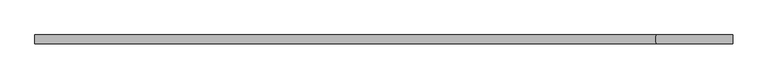
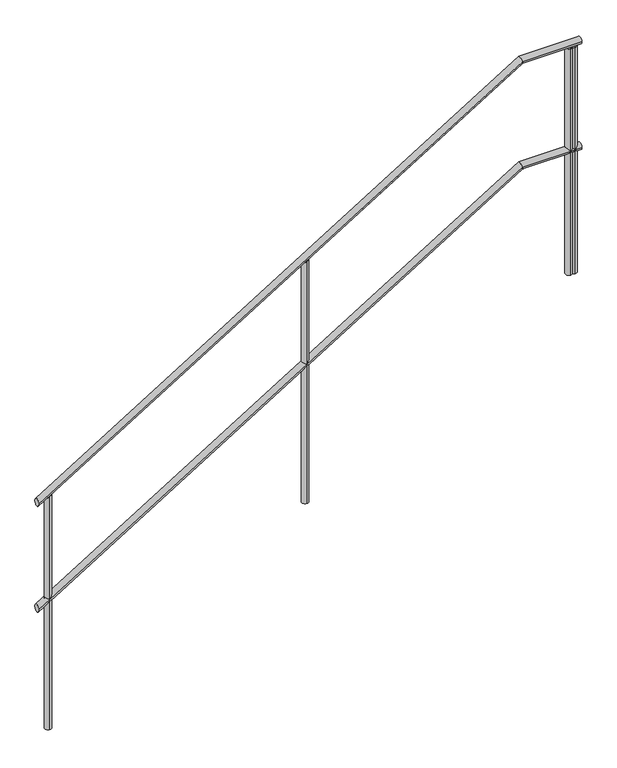
"""IFC4 building model written with IfcOpenShell, lengths in millimetres: railing geometry."""

from ifc_helpers import new_model, si_unit, point, frame, frame_2d, origin, place, context, project, spatial, circle_curve, ellipse_curve, trimmed, segment, composite_curve, outline, extrude, source, transform, mapped, element, save
from ifc_brep_helpers import plane_surface, cylinder_surface, advanced_brep


def railing_2ca88775(model_context):
    return source(origin(), model_context, "Body", "SolidModel", [
        advanced_brep(
        [(71751.0, -5865.7674116, -450.9609787), (71751.0, -5835.7674116, -450.9609787), (73915.2567855, -5835.7674116, 885.0), (73915.2567855, -5865.7674116, 885.0), (74181.0, -5865.7674116, 885.0), (74181.0, -5835.7674116, 885.0)],
        [
            (0, 1, ellipse_curve(frame((71751.0, -5850.7674116, -450.9609787), z_axis=(-1.0, 0.0, 0.0), x_axis=(0.0, 0.0, -1.0)), 17.6276454, 15.0)),
            (1, 0, ellipse_curve(frame((71751.0, -5850.7674116, -450.9609787), z_axis=(-1.0, 0.0, 0.0), x_axis=(0.0, 0.0, -1.0)), 17.6276454, 15.0)),
            (1, 2),
            (2, 3, ellipse_curve(frame((73915.2567855, -5850.7674116, 885.0), z_axis=(-0.9620125025549409, 0.0, -0.27300539358770864), x_axis=(0.27300539358770803, 0.0, -0.9620125025549412)), 15.5923129, 15.0)),
            (3, 0),
            (3, 2, ellipse_curve(frame((73915.2567855, -5850.7674116, 885.0), z_axis=(-0.9620125025549409, 0.0, -0.27300539358770864), x_axis=(0.27300539358770803, 0.0, -0.9620125025549412)), 15.5923129, 15.0)),
            (4, 5, circle_curve(frame((74181.0, -5850.7674116, 885.0), z_axis=(1.0, 0.0, 0.0), x_axis=(0.0, 1.0, 0.0)), 15.0)),
            (5, 4, circle_curve(frame((74181.0, -5850.7674116, 885.0), z_axis=(1.0, 0.0, 0.0), x_axis=(0.0, 1.0, 0.0)), 15.0)),
            (2, 5),
            (4, 3),
        ],
        [
            plane_surface(frame((71751.0, -5850.7674116, -433.3333333), z_axis=(-1.0, 0.0, 0.0), x_axis=(0.0, 1.0, 0.0))),
            cylinder_surface(frame((71758.8790381, -5850.7674116, -446.097375), z_axis=(-0.8509361101440404, 0.0, -0.5252692037926168), x_axis=(0.0, 1.0, 0.0)), 15.0),
            plane_surface(frame((74181.0, -5850.7674116, 900.0), z_axis=(1.0, 0.0, 0.0), x_axis=(0.0, 1.0, 0.0))),
            cylinder_surface(frame((73911.0, -5850.7674116, 885.0), z_axis=(-1.0, 0.0, 0.0), x_axis=(0.0, 1.0, 0.0)), 15.0),
        ],
        [
            (0, [[1, 2]]),
            (1, [[-2, 3, 4, 5]]),
            (1, [[-1, -5, 6, -3]]),
            (2, [[7, 8]]),
            (3, [[-4, 9, -7, 10]]),
            (3, [[-6, -10, -8, -9]]),
        ],
    ),
        advanced_brep(
        [(71751.0, -5865.7674116, 49.0390213), (71751.0, -5835.7674116, 49.0390213), (73915.2567855, -5835.7674116, 1385.0), (73915.2567855, -5865.7674116, 1385.0), (74181.0, -5865.7674116, 1385.0), (74181.0, -5835.7674116, 1385.0)],
        [
            (0, 1, ellipse_curve(frame((71751.0, -5850.7674116, 49.0390213), z_axis=(-1.0, 0.0, 0.0), x_axis=(0.0, 0.0, -1.0)), 17.6276454, 15.0)),
            (1, 0, ellipse_curve(frame((71751.0, -5850.7674116, 49.0390213), z_axis=(-1.0, 0.0, 0.0), x_axis=(0.0, 0.0, -1.0)), 17.6276454, 15.0)),
            (1, 2),
            (2, 3, ellipse_curve(frame((73915.2567855, -5850.7674116, 1385.0), z_axis=(-0.9620125025549409, 0.0, -0.27300539358770864), x_axis=(0.27300539358770803, 0.0, -0.9620125025549412)), 15.5923129, 15.0)),
            (3, 0),
            (3, 2, ellipse_curve(frame((73915.2567855, -5850.7674116, 1385.0), z_axis=(-0.9620125025549409, 0.0, -0.27300539358770864), x_axis=(0.27300539358770803, 0.0, -0.9620125025549412)), 15.5923129, 15.0)),
            (4, 5, circle_curve(frame((74181.0, -5850.7674116, 1385.0), z_axis=(1.0, 0.0, 0.0), x_axis=(0.0, 1.0, 0.0)), 15.0)),
            (5, 4, circle_curve(frame((74181.0, -5850.7674116, 1385.0), z_axis=(1.0, 0.0, 0.0), x_axis=(0.0, 1.0, 0.0)), 15.0)),
            (2, 5),
            (4, 3),
        ],
        [
            plane_surface(frame((71751.0, -5850.7674116, 66.6666667), z_axis=(-1.0, 0.0, 0.0), x_axis=(0.0, 1.0, 0.0))),
            cylinder_surface(frame((71758.8790381, -5850.7674116, 53.902625), z_axis=(-0.8509361101440404, 0.0, -0.5252692037926168), x_axis=(0.0, 1.0, 0.0)), 15.0),
            plane_surface(frame((74181.0, -5850.7674116, 1400.0), z_axis=(1.0, 0.0, 0.0), x_axis=(0.0, 1.0, 0.0))),
            cylinder_surface(frame((73911.0, -5850.7674116, 1385.0), z_axis=(-1.0, 0.0, 0.0), x_axis=(0.0, 1.0, 0.0)), 15.0),
        ],
        [
            (0, [[1, 2]]),
            (1, [[-2, 3, 4, 5]]),
            (1, [[-1, -5, 6, -3]]),
            (2, [[7, 8]]),
            (3, [[-4, 9, -7, 10]]),
            (3, [[-6, -10, -8, -9]]),
        ],
    ),
        extrude(outline(composite_curve([segment(trimmed(circle_curve(frame_2d((74151.0, -5850.7674116)), 15.0), [point((74151.0, -5865.7674116))], [point((74151.0, -5835.7674116))], False, "CARTESIAN"), True, "CONTINUOUS"), segment(trimmed(circle_curve(frame_2d((74151.0, -5850.7674116)), 15.0), [point((74151.0, -5835.7674116))], [point((74151.0, -5865.7674116))], False, "CARTESIAN"), True, "CONTINUOUS")], self_intersect=False)), frame((0.0, 0.0, 300.0), z_axis=(0.0, 0.0, 1.0), x_axis=(1.0, 0.0, 0.0)), (0.0, 0.0, 1.0), 1070.0),
        advanced_brep(
        [(72951.0, -5835.7674116, 777.4074074), (72951.0, -5865.7674116, 777.4074074), (72951.0, -5865.7674116, -366.6666667), (72951.0, -5835.7674116, -366.6666667)],
        [
            (0, 1, ellipse_curve(frame((72951.0, -5850.7674116, 777.4074074), z_axis=(0.5252692037926167, 0.0, -0.8509361101440406), x_axis=(0.8509361101440406, 0.0, 0.5252692037926162)), 17.6276454, 15.0)),
            (1, 2),
            (2, 3, circle_curve(frame((72951.0, -5850.7674116, -366.6666667), z_axis=(0.0, 0.0, 1.0), x_axis=(0.0, -1.0, 0.0)), 15.0)),
            (3, 0),
            (3, 2, circle_curve(frame((72951.0, -5850.7674116, -366.6666667), z_axis=(0.0, 0.0, 1.0), x_axis=(0.0, -1.0, 0.0)), 15.0)),
            (1, 0, ellipse_curve(frame((72951.0, -5850.7674116, 777.4074074), z_axis=(0.5252692037926167, 0.0, -0.8509361101440406), x_axis=(0.8509361101440406, 0.0, 0.5252692037926162)), 17.6276454, 15.0)),
        ],
        [
            cylinder_surface(frame((72951.0, -5850.7674116, -466.6666667), z_axis=(0.0, 0.0, 1.0), x_axis=(0.0, -1.0, 0.0)), 15.0),
            plane_surface(frame((72976.0, -5875.7674116, 792.8395062), z_axis=(-0.5252692037926167, 0.0, 0.8509361101440406), x_axis=(0.0, 1.0, 0.0))),
            plane_surface(frame((72926.0, -5875.7674116, -366.6666667), z_axis=(0.0, 0.0, -1.0), x_axis=(0.0, 1.0, 0.0))),
        ],
        [
            (0, [[1, 2, 3, 4]]),
            (0, [[5, -2, 6, -4]]),
            (1, [[-6, -1]]),
            (2, [[-5, -3]]),
        ],
    ),
        extrude(outline(composite_curve([segment(trimmed(circle_curve(frame_2d((74131.0, -5850.7674116)), 15.0), [point((74131.0, -5865.7674116))], [point((74131.0, -5835.7674116))], False, "CARTESIAN"), True, "CONTINUOUS"), segment(trimmed(circle_curve(frame_2d((74131.0, -5850.7674116)), 15.0), [point((74131.0, -5835.7674116))], [point((74131.0, -5865.7674116))], False, "CARTESIAN"), True, "CONTINUOUS")], self_intersect=False)), frame((0.0, 0.0, 300.0), z_axis=(0.0, 0.0, 1.0), x_axis=(1.0, 0.0, 0.0)), (0.0, 0.0, 1.0), 1070.0),
        advanced_brep(
        [(71801.0, -5835.7674116, 67.5308642), (71801.0, -5865.7674116, 67.5308642), (71801.0, -5865.7674116, -1033.3333333), (71801.0, -5835.7674116, -1033.3333333)],
        [
            (0, 1, ellipse_curve(frame((71801.0, -5850.7674116, 67.5308642), z_axis=(0.5252692037926167, 0.0, -0.8509361101440406), x_axis=(0.8509361101440406, 0.0, 0.5252692037926162)), 17.6276454, 15.0)),
            (1, 2),
            (2, 3, circle_curve(frame((71801.0, -5850.7674116, -1033.3333333), z_axis=(0.0, 0.0, 1.0), x_axis=(0.0, -1.0, 0.0)), 15.0)),
            (3, 0),
            (3, 2, circle_curve(frame((71801.0, -5850.7674116, -1033.3333333), z_axis=(0.0, 0.0, 1.0), x_axis=(0.0, -1.0, 0.0)), 15.0)),
            (1, 0, ellipse_curve(frame((71801.0, -5850.7674116, 67.5308642), z_axis=(0.5252692037926167, 0.0, -0.8509361101440406), x_axis=(0.8509361101440406, 0.0, 0.5252692037926162)), 17.6276454, 15.0)),
        ],
        [
            cylinder_surface(frame((71801.0, -5850.7674116, -1133.3333333), z_axis=(0.0, 0.0, 1.0), x_axis=(0.0, -1.0, 0.0)), 15.0),
            plane_surface(frame((71826.0, -5875.7674116, 82.962963), z_axis=(-0.5252692037926167, 0.0, 0.8509361101440406), x_axis=(0.0, 1.0, 0.0))),
            plane_surface(frame((71776.0, -5875.7674116, -1033.3333333), z_axis=(0.0, 0.0, -1.0), x_axis=(0.0, 1.0, 0.0))),
        ],
        [
            (0, [[1, 2, 3, 4]]),
            (0, [[5, -2, 6, -4]]),
            (1, [[-6, -1]]),
            (2, [[-5, -3]]),
        ],
    ),
    ])


if __name__ == "__main__":
    model = new_model("IFC4")
    model_context = context("Model", 3, world=origin())
    ifc_project = project(units=[si_unit("LENGTHUNIT", "METRE", prefix="MILLI")], contexts=[model_context])
    site = spatial("IfcSite", under=ifc_project)
    building = spatial("IfcBuilding", under=site)
    placement = place(None, origin())
    railing_shape = railing_2ca88775(model_context)
    element("IfcRailing", 1, at=placement, inside=building, context=model_context, shape_type="MappedRepresentation", body=[
        mapped(railing_shape, transform((0.0, 0.0, 0.0), x_axis=(1.0, 0.0, 0.0), y_axis=(0.0, 1.0, 0.0), z_axis=(0.0, 0.0, 1.0))),
    ])
    save(model, "model.ifc")
